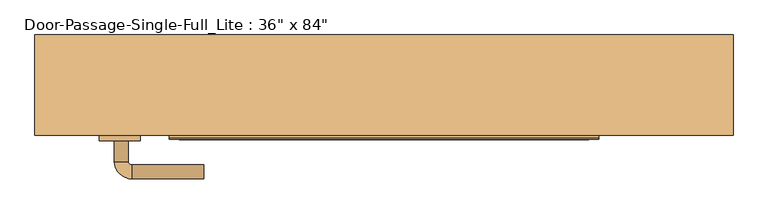
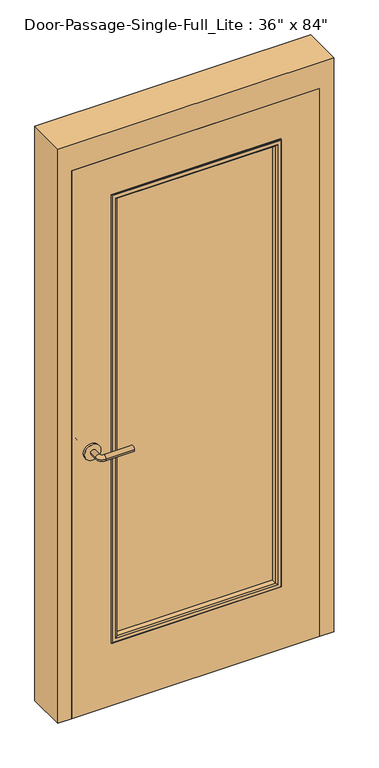
"""IFC4 building model written with IfcOpenShell, lengths in millimetres: door geometry."""

from ifc_helpers import new_model, si_unit, point, frame, frame_2d, origin, place, context, project, spatial, polyline, circle_curve, ellipse_curve, trimmed, segment, composite_curve, outline, extrude, faceted_brep, source, transform, mapped, element, save
from ifc_brep_helpers import plane_surface, cylinder_surface, revolved_surface, advanced_brep


def door_58f93f42(model_context):
    return source(origin(), model_context, "Body", "SolidModel", [
        advanced_brep(
        [(-392.190625, 1.65, 1016.0), (-372.190625, 1.65, 1016.0), (-392.190625, 31.65, 1016.0), (-372.190625, 31.65, 1016.0), (-367.190625, 36.65, 1016.0), (-367.190625, 56.65, 1016.0), (-262.190625, 56.65, 1016.0), (-262.190625, 36.65, 1016.0)],
        [
            (0, 1, circle_curve(frame((-382.190625, 1.65, 1016.0), z_axis=(0.0, -1.0, 0.0), x_axis=(1.0, 0.0, 0.0)), 10.0)),
            (1, 0, circle_curve(frame((-382.190625, 1.65, 1016.0), z_axis=(0.0, -1.0, 0.0), x_axis=(1.0, 0.0, 0.0)), 10.0)),
            (0, 2),
            (2, 3, circle_curve(frame((-382.190625, 31.65, 1016.0), z_axis=(0.0, -1.0, 0.0), x_axis=(1.0, 0.0, 0.0)), 10.0)),
            (3, 1),
            (3, 2, circle_curve(frame((-382.190625, 31.65, 1016.0), z_axis=(0.0, -1.0, 0.0), x_axis=(1.0, 0.0, 0.0)), 10.0)),
            (4, 3, circle_curve(frame((-367.190625, 31.65, 1016.0), z_axis=(0.0, 0.0, 1.0), x_axis=(-1.0, 0.0, 0.0)), 5.0)),
            (2, 5, circle_curve(frame((-367.190625, 31.65, 1016.0), z_axis=(0.0, 0.0, -1.0), x_axis=(-1.0, 0.0, 0.0)), 25.0)),
            (5, 4, circle_curve(frame((-367.190625, 46.65, 1016.0), z_axis=(-1.0, 0.0, 0.0), x_axis=(0.0, -1.0, 0.0)), 10.0)),
            (4, 5, circle_curve(frame((-367.190625, 46.65, 1016.0), z_axis=(-1.0, 0.0, 0.0), x_axis=(0.0, -1.0, 0.0)), 10.0)),
            (6, 7, circle_curve(frame((-262.190625, 46.65, 1016.0), z_axis=(1.0, 0.0, 0.0), x_axis=(0.0, -1.0, 0.0)), 10.0)),
            (7, 6, circle_curve(frame((-262.190625, 46.65, 1016.0), z_axis=(1.0, 0.0, 0.0), x_axis=(0.0, -1.0, 0.0)), 10.0)),
            (5, 6),
            (7, 4),
        ],
        [
            plane_surface(frame((-382.190625, 1.65, 1016.0), z_axis=(0.0, -1.0, 0.0), x_axis=(0.0, 0.0, 1.0))),
            cylinder_surface(frame((-382.190625, 1.65, 1016.0), z_axis=(0.0, -1.0, 0.0), x_axis=(1.0, 0.0, 0.0)), 10.0),
            revolved_surface(trimmed(ellipse_curve(frame((-382.190625, 31.65, 1016.0), z_axis=(0.0, -1.0, 0.0), x_axis=(1.0, 0.0, 0.0)), 10.0, 10.0), [point((-392.190625, 31.65, 1016.0))], [point((-372.190625, 31.65, 1016.0))], True, "CARTESIAN"), (-367.190625, 31.65, 1016.0), (0.0, 0.0, -1.0)),
            revolved_surface(trimmed(ellipse_curve(frame((-382.190625, 31.65, 1016.0), z_axis=(0.0, -1.0, 0.0), x_axis=(1.0, 0.0, 0.0)), 10.0, 10.0), [point((-372.190625, 31.65, 1016.0))], [point((-392.190625, 31.65, 1016.0))], True, "CARTESIAN"), (-367.190625, 31.65, 1016.0), (0.0, 0.0, -1.0)),
            plane_surface(frame((-262.190625, 46.65, 1016.0), z_axis=(1.0, 0.0, 0.0), x_axis=(0.0, 0.0, 1.0))),
            cylinder_surface(frame((-367.190625, 46.65, 1016.0), z_axis=(-1.0, 0.0, 0.0), x_axis=(0.0, -1.0, 0.0)), 10.0),
        ],
        [
            (0, [[1, 2]]),
            (1, [[-1, 3, 4, 5]]),
            (1, [[-2, -5, 6, -3]]),
            (2, [[7, -4, 8, 9]]),
            (3, [[-8, -6, -7, 10]]),
            (4, [[11, 12]]),
            (5, [[-9, 13, -12, 14]]),
            (5, [[-10, -14, -11, -13]]),
        ],
    ),
        extrude(outline(composite_curve([segment(trimmed(circle_curve(frame_2d((1016.0, -384.690625)), 30.0), [point((1016.0, -414.690625))], [point((1016.0, -354.690625))], False, "CARTESIAN"), True, "CONTINUOUS"), segment(trimmed(circle_curve(frame_2d((1016.0, -384.690625)), 30.0), [point((1016.0, -354.690625))], [point((1016.0, -414.690625))], False, "CARTESIAN"), True, "CONTINUOUS")], self_intersect=False)), frame((0.0, -6.35, 0.0), z_axis=(0.0, 1.0, 0.0), x_axis=(0.0, 0.0, 1.0)), (0.0, 0.0, 1.0), 8.0),
        advanced_brep(
        [(-392.190625, -58.8, 1016.0), (-372.190625, -58.8, 1016.0), (-372.190625, -88.8, 1016.0), (-392.190625, -88.8, 1016.0), (-367.190625, -93.8, 1016.0), (-367.190625, -113.8, 1016.0), (-262.190625, -113.8, 1016.0), (-262.190625, -93.8, 1016.0)],
        [
            (0, 1, circle_curve(frame((-382.190625, -58.8, 1016.0), z_axis=(0.0, 1.0, 0.0), x_axis=(1.0, 0.0, 0.0)), 10.0)),
            (1, 0, circle_curve(frame((-382.190625, -58.8, 1016.0), z_axis=(0.0, 1.0, 0.0), x_axis=(1.0, 0.0, 0.0)), 10.0)),
            (1, 2),
            (2, 3, circle_curve(frame((-382.190625, -88.8, 1016.0), z_axis=(0.0, 1.0, 0.0), x_axis=(1.0, 0.0, 0.0)), 10.0)),
            (3, 0),
            (3, 2, circle_curve(frame((-382.190625, -88.8, 1016.0), z_axis=(0.0, 1.0, 0.0), x_axis=(1.0, 0.0, 0.0)), 10.0)),
            (4, 5, circle_curve(frame((-367.190625, -103.8, 1016.0), z_axis=(-1.0, 0.0, 0.0), x_axis=(0.0, 1.0, 0.0)), 10.0)),
            (5, 3, circle_curve(frame((-367.190625, -88.8, 1016.0), z_axis=(0.0, 0.0, -1.0), x_axis=(-1.0, 0.0, 0.0)), 25.0)),
            (2, 4, circle_curve(frame((-367.190625, -88.8, 1016.0), z_axis=(0.0, 0.0, 1.0), x_axis=(-1.0, 0.0, 0.0)), 5.0)),
            (5, 4, circle_curve(frame((-367.190625, -103.8, 1016.0), z_axis=(-1.0, 0.0, 0.0), x_axis=(0.0, 1.0, 0.0)), 10.0)),
            (6, 7, circle_curve(frame((-262.190625, -103.8, 1016.0), z_axis=(1.0, 0.0, 0.0), x_axis=(0.0, 1.0, 0.0)), 10.0)),
            (7, 6, circle_curve(frame((-262.190625, -103.8, 1016.0), z_axis=(1.0, 0.0, 0.0), x_axis=(0.0, 1.0, 0.0)), 10.0)),
            (4, 7),
            (6, 5),
        ],
        [
            plane_surface(frame((-382.190625, -58.8, 1016.0), z_axis=(0.0, 1.0, 0.0), x_axis=(0.0, 0.0, 1.0))),
            cylinder_surface(frame((-382.190625, -58.8, 1016.0), z_axis=(0.0, 1.0, 0.0), x_axis=(1.0, 0.0, 0.0)), 10.0),
            revolved_surface(trimmed(ellipse_curve(frame((-382.190625, -88.8, 1016.0), z_axis=(0.0, -1.0, 0.0), x_axis=(1.0, 0.0, 0.0)), 10.0, 10.0), [point((-392.190625, -88.8, 1016.0))], [point((-372.190625, -88.8, 1016.0))], True, "CARTESIAN"), (-367.190625, -88.8, 1016.0), (0.0, 0.0, -1.0)),
            revolved_surface(trimmed(ellipse_curve(frame((-382.190625, -88.8, 1016.0), z_axis=(0.0, -1.0, 0.0), x_axis=(1.0, 0.0, 0.0)), 10.0, 10.0), [point((-372.190625, -88.8, 1016.0))], [point((-392.190625, -88.8, 1016.0))], True, "CARTESIAN"), (-367.190625, -88.8, 1016.0), (0.0, 0.0, -1.0)),
            plane_surface(frame((-262.190625, -103.8, 1016.0), z_axis=(1.0, 0.0, 0.0), x_axis=(0.0, 0.0, 1.0))),
            cylinder_surface(frame((-367.190625, -103.8, 1016.0), z_axis=(-1.0, 0.0, 0.0), x_axis=(0.0, 1.0, 0.0)), 10.0),
        ],
        [
            (0, [[1, 2]]),
            (1, [[3, 4, 5, -2]]),
            (1, [[-5, 6, -3, -1]]),
            (2, [[7, 8, -4, 9]]),
            (3, [[10, -9, -6, -8]]),
            (4, [[11, 12]]),
            (5, [[13, -11, 14, -7]]),
            (5, [[-14, -12, -13, -10]]),
        ],
    ),
        extrude(outline(composite_curve([segment(trimmed(circle_curve(frame_2d((1016.0, -384.690625)), 30.0), [point((1016.0, -414.690625))], [point((1016.0, -354.690625))], False, "CARTESIAN"), True, "CONTINUOUS"), segment(trimmed(circle_curve(frame_2d((1016.0, -384.690625)), 30.0), [point((1016.0, -354.690625))], [point((1016.0, -414.690625))], False, "CARTESIAN"), True, "CONTINUOUS")], self_intersect=False)), frame((0.0, -58.8, 0.0), z_axis=(0.0, 1.0, 0.0), x_axis=(0.0, 0.0, 1.0)), (0.0, 0.0, 1.0), 8.0),
        extrude(outline(polyline([(304.8, -25.4), (304.8, -31.75), (-304.8, -31.75), (-304.8, -25.4), (304.8, -25.4)])), frame((0.0, 0.0, 254.0), z_axis=(0.0, 0.0, 1.0), x_axis=(1.0, 0.0, 0.0)), (0.0, 0.0, 1.0), 1727.2),
        faceted_brep([(457.2, -1.5875, 0.0), (441.325, -1.5875, 0.0), (441.325, 46.0375, 0.0), (457.2, 46.0375, 0.0), (457.2, 95.25, 0.0), (508.0, 95.25, 0.0), (508.0, -50.8, 0.0), (457.2, -50.8, 0.0), (457.2, -50.8, 2133.6), (457.2, -1.5875, 2133.6), (508.0, -50.8, 2235.2), (-508.0, -50.8, 2235.2), (-508.0, -50.8, 0.0), (-457.2, -50.8, 0.0), (-457.2, -50.8, 2133.6), (508.0, 95.25, 2235.2), (457.2, 95.25, 2133.6), (-457.2, 95.25, 2133.6), (-457.2, 95.25, 0.0), (-508.0, 95.25, 0.0), (-508.0, 95.25, 2235.2), (457.2, 46.0375, 2133.6), (441.325, 46.0375, 2117.725), (-441.325, 46.0375, 2117.725), (-441.325, 46.0375, 0.0), (-457.2, 46.0375, 0.0), (-457.2, 46.0375, 2133.6), (441.325, -1.5875, 2117.725), (-457.2, -1.5875, 2133.6), (-457.2, -1.5875, 0.0), (-441.325, -1.5875, 0.0), (-441.325, -1.5875, 2117.725)], [[[0, 1, 2, 3, 4, 5, 6, 7]], [[7, 8, 9, 0]], [[6, 10, 11, 12, 13, 14, 8, 7]], [[5, 15, 10, 6]], [[4, 16, 17, 18, 19, 20, 15, 5]], [[3, 21, 16, 4]], [[2, 22, 23, 24, 25, 26, 21, 3]], [[1, 27, 22, 2]], [[0, 9, 28, 29, 30, 31, 27, 1]], [[8, 14, 28, 9]], [[16, 21, 26, 17]], [[22, 27, 31, 23]], [[12, 19, 18, 25, 24, 30, 29, 13]], [[13, 29, 28, 14]], [[11, 20, 19, 12]], [[17, 26, 25, 18]], [[23, 31, 30, 24]], [[15, 20, 11, 10]]]),
        extrude(outline(polyline([(2133.6, -457.2), (0.0, -457.2), (0.0, 457.2), (2133.6, 457.2), (2133.6, -457.2)]), holes=[polyline([(1981.2, -304.8), (1981.2, 304.8), (254.0, 304.8), (254.0, -304.8), (1981.2, -304.8)])]), frame((0.0, -50.8, 0.0), z_axis=(0.0, 1.0, 0.0), x_axis=(0.0, 0.0, 1.0)), (0.0, 0.0, 1.0), 44.45),
        advanced_brep(
        [(-304.8, -31.75, 1981.2), (-304.8, -31.75, 254.0), (-304.8, -50.8, 254.0), (-304.8, -50.8, 1981.2), (-292.8, -51.8, 1969.2), (-292.8, -51.8, 266.0), (-292.8, -31.75, 266.0), (-292.8, -31.75, 1969.2), (-297.8, -56.8, 1974.2), (-297.8, -56.8, 261.0), (-312.8, -54.8, 1989.2), (-312.8, -54.8, 246.0), (-310.8, -56.8, 248.0), (-310.8, -56.8, 1987.2), (-312.8, -50.8, 1989.2), (-312.8, -50.8, 246.0), (304.8, -31.75, 254.0), (304.8, -50.8, 254.0), (292.8, -51.8, 266.0), (292.8, -31.75, 266.0), (297.8, -56.8, 261.0), (312.8, -54.8, 246.0), (310.8, -56.8, 248.0), (312.8, -50.8, 246.0), (304.8, -31.75, 1981.2), (304.8, -50.8, 1981.2), (292.8, -51.8, 1969.2), (292.8, -31.75, 1969.2), (297.8, -56.8, 1974.2), (312.8, -54.8, 1989.2), (310.8, -56.8, 1987.2), (312.8, -50.8, 1989.2)],
        [
            (0, 1),
            (1, 2),
            (2, 3),
            (3, 0),
            (4, 5),
            (5, 6),
            (6, 7),
            (7, 4),
            (8, 9),
            (9, 5, ellipse_curve(frame((-297.8, -51.8, 261.0), z_axis=(-0.7071067811865475, 0.0, 0.7071067811865475), x_axis=(0.7071067811865474, 0.0, 0.7071067811865476)), 7.0710678, 5.0)),
            (4, 8, ellipse_curve(frame((-297.8, -51.8, 1974.2), z_axis=(-0.7071067811865475, 0.0, -0.7071067811865475), x_axis=(-0.7071067811865474, 0.0, 0.7071067811865476)), 7.0710678, 5.0)),
            (10, 11),
            (11, 12, ellipse_curve(frame((-310.8, -54.8, 248.0), z_axis=(-0.7071067811865475, 0.0, 0.7071067811865475), x_axis=(0.7071067811865474, 0.0, 0.7071067811865476)), 2.8284271, 2.0)),
            (12, 13),
            (13, 10, ellipse_curve(frame((-310.8, -54.8, 1987.2), z_axis=(-0.7071067811865475, 0.0, -0.7071067811865475), x_axis=(-0.7071067811865474, 0.0, 0.7071067811865476)), 2.8284271, 2.0)),
            (14, 15),
            (15, 11),
            (10, 14),
            (1, 16),
            (16, 17),
            (17, 2),
            (5, 18),
            (18, 19),
            (19, 6),
            (9, 20),
            (20, 18, ellipse_curve(frame((297.8, -51.8, 261.0), z_axis=(-0.7071067811865475, 0.0, -0.7071067811865475), x_axis=(-0.7071067811865476, 0.0, 0.7071067811865474)), 7.0710678, 5.0)),
            (11, 21),
            (21, 22, ellipse_curve(frame((310.8, -54.8, 248.0), z_axis=(-0.7071067811865475, 0.0, -0.7071067811865475), x_axis=(-0.7071067811865476, 0.0, 0.7071067811865474)), 2.8284271, 2.0)),
            (22, 12),
            (15, 23),
            (23, 21),
            (16, 24),
            (24, 25),
            (25, 17),
            (18, 26),
            (26, 27),
            (27, 19),
            (20, 28),
            (28, 26, ellipse_curve(frame((297.8, -51.8, 1974.2), z_axis=(0.7071067811865475, 0.0, -0.7071067811865475), x_axis=(-0.7071067811865474, 0.0, -0.7071067811865476)), 7.0710678, 5.0)),
            (21, 29),
            (29, 30, ellipse_curve(frame((310.8, -54.8, 1987.2), z_axis=(0.7071067811865475, 0.0, -0.7071067811865475), x_axis=(-0.7071067811865474, 0.0, -0.7071067811865476)), 2.8284271, 2.0)),
            (30, 22),
            (23, 31),
            (31, 29),
            (14, 31),
            (25, 3),
            (24, 0),
            (27, 7),
            (26, 4),
            (28, 8),
            (30, 13),
            (29, 10),
        ],
        [
            plane_surface(frame((-304.8, -50.8, 1981.2), z_axis=(-1.0, 0.0, 0.0), x_axis=(0.0, 0.0, -1.0))),
            plane_surface(frame((-292.8, -31.75, 1969.2), z_axis=(1.0, 0.0, 0.0), x_axis=(0.0, 0.0, -1.0))),
            cylinder_surface(frame((-297.8, -51.8, 1981.2), z_axis=(0.0, 0.0, 1.0), x_axis=(-1.0, 0.0, 0.0)), 5.0),
            cylinder_surface(frame((-310.8, -54.8, 1981.2), z_axis=(0.0, 0.0, 1.0), x_axis=(-1.0, 0.0, 0.0)), 2.0),
            plane_surface(frame((-312.8, -54.8, 1989.2), z_axis=(-1.0, 0.0, 0.0), x_axis=(0.0, 0.0, -1.0))),
            plane_surface(frame((-304.8, -50.8, 254.0), z_axis=(0.0, 0.0, -1.0), x_axis=(1.0, 0.0, 0.0))),
            plane_surface(frame((-292.8, -31.75, 266.0), z_axis=(0.0, 0.0, 1.0), x_axis=(1.0, 0.0, 0.0))),
            cylinder_surface(frame((-304.8, -51.8, 261.0), z_axis=(-1.0, 0.0, 0.0), x_axis=(0.0, 0.0, -1.0)), 5.0),
            cylinder_surface(frame((-304.8, -54.8, 248.0), z_axis=(-1.0, 0.0, 0.0), x_axis=(0.0, 0.0, -1.0)), 2.0),
            plane_surface(frame((-312.8, -54.8, 246.0), z_axis=(0.0, 0.0, -1.0), x_axis=(1.0, 0.0, 0.0))),
            plane_surface(frame((304.8, -50.8, 254.0), z_axis=(1.0, 0.0, 0.0), x_axis=(0.0, 0.0, 1.0))),
            plane_surface(frame((292.8, -31.75, 266.0), z_axis=(-1.0, 0.0, 0.0), x_axis=(0.0, 0.0, 1.0))),
            cylinder_surface(frame((297.8, -51.8, 254.0), z_axis=(0.0, 0.0, -1.0), x_axis=(1.0, 0.0, 0.0)), 5.0),
            cylinder_surface(frame((310.8, -54.8, 254.0), z_axis=(0.0, 0.0, -1.0), x_axis=(1.0, 0.0, 0.0)), 2.0),
            plane_surface(frame((312.8, -54.8, 246.0), z_axis=(1.0, 0.0, 0.0), x_axis=(0.0, 0.0, 1.0))),
            plane_surface(frame((312.8, -50.8, 1989.2), z_axis=(0.0, 1.0, 0.0), x_axis=(-1.0, 0.0, 0.0))),
            plane_surface(frame((304.8, -50.8, 1981.2), z_axis=(0.0, 0.0, 1.0), x_axis=(-1.0, 0.0, 0.0))),
            plane_surface(frame((304.8, -31.75, 1981.2), z_axis=(0.0, 1.0, 0.0), x_axis=(-1.0, 0.0, 0.0))),
            plane_surface(frame((292.8, -31.75, 1969.2), z_axis=(0.0, 0.0, -1.0), x_axis=(-1.0, 0.0, 0.0))),
            cylinder_surface(frame((304.8, -51.8, 1974.2), z_axis=(1.0, 0.0, 0.0), x_axis=(0.0, 0.0, 1.0)), 5.0),
            plane_surface(frame((297.8, -56.8, 1974.2), z_axis=(0.0, -1.0, 0.0), x_axis=(-1.0, 0.0, 0.0))),
            cylinder_surface(frame((304.8, -54.8, 1987.2), z_axis=(1.0, 0.0, 0.0), x_axis=(0.0, 0.0, 1.0)), 2.0),
            plane_surface(frame((312.8, -54.8, 1989.2), z_axis=(0.0, 0.0, 1.0), x_axis=(-1.0, 0.0, 0.0))),
        ],
        [
            (0, [[1, 2, 3, 4]]),
            (1, [[5, 6, 7, 8]]),
            (2, [[9, 10, -5, 11]]),
            (3, [[12, 13, 14, 15]]),
            (4, [[16, 17, -12, 18]]),
            (5, [[19, 20, 21, -2]]),
            (6, [[22, 23, 24, -6]]),
            (7, [[25, 26, -22, -10]]),
            (8, [[27, 28, 29, -13]]),
            (9, [[30, 31, -27, -17]]),
            (10, [[32, 33, 34, -20]]),
            (11, [[35, 36, 37, -23]]),
            (12, [[38, 39, -35, -26]]),
            (13, [[40, 41, 42, -28]]),
            (14, [[43, 44, -40, -31]]),
            (15, [[-16, 45, -43, -30], [-3, -21, -34, 46]]),
            (16, [[47, -4, -46, -33]]),
            (17, [[-1, -47, -32, -19], [-7, -24, -37, 48]]),
            (18, [[49, -8, -48, -36]]),
            (19, [[50, -11, -49, -39]]),
            (20, [[-14, -29, -42, 51], [-9, -50, -38, -25]]),
            (21, [[52, -15, -51, -41]]),
            (22, [[-45, -18, -52, -44]]),
        ],
    ),
        advanced_brep(
        [(-304.8, -25.4, 254.0), (-304.8, -25.4, 1981.2), (-304.8, -6.35, 1981.2), (-304.8, -6.35, 254.0), (-292.8, -5.35, 266.0), (-292.8, -5.35, 1969.2), (-292.8, -25.4, 1969.2), (-292.8, -25.4, 266.0), (-297.8, -0.35, 261.0), (-297.8, -0.35, 1974.2), (-312.8, -2.35, 246.0), (-312.8, -2.35, 1989.2), (-310.8, -0.35, 1987.2), (-310.8, -0.35, 248.0), (-312.8, -6.35, 246.0), (-312.8, -6.35, 1989.2), (304.8, -25.4, 1981.2), (304.8, -6.35, 1981.2), (292.8, -5.35, 1969.2), (292.8, -25.4, 1969.2), (297.8, -0.35, 1974.2), (312.8, -2.35, 1989.2), (310.8, -0.35, 1987.2), (312.8, -6.35, 1989.2), (304.8, -25.4, 254.0), (304.8, -6.35, 254.0), (292.8, -5.35, 266.0), (292.8, -25.4, 266.0), (297.8, -0.35, 261.0), (312.8, -2.35, 246.0), (310.8, -0.35, 248.0), (312.8, -6.35, 246.0)],
        [
            (0, 1),
            (1, 2),
            (2, 3),
            (3, 0),
            (4, 5),
            (5, 6),
            (6, 7),
            (7, 4),
            (8, 9),
            (9, 5, ellipse_curve(frame((-297.8, -5.35, 1974.2), z_axis=(-0.7071067811865475, 0.0, -0.7071067811865475), x_axis=(0.7071067811865474, 0.0, -0.7071067811865476)), 7.0710678, 5.0)),
            (4, 8, ellipse_curve(frame((-297.8, -5.35, 261.0), z_axis=(-0.7071067811865475, 0.0, 0.7071067811865475), x_axis=(-0.7071067811865474, 0.0, -0.7071067811865476)), 7.0710678, 5.0)),
            (10, 11),
            (11, 12, ellipse_curve(frame((-310.8, -2.35, 1987.2), z_axis=(-0.7071067811865475, 0.0, -0.7071067811865475), x_axis=(0.7071067811865474, 0.0, -0.7071067811865476)), 2.8284271, 2.0)),
            (12, 13),
            (13, 10, ellipse_curve(frame((-310.8, -2.35, 248.0), z_axis=(-0.7071067811865475, 0.0, 0.7071067811865475), x_axis=(-0.7071067811865474, 0.0, -0.7071067811865476)), 2.8284271, 2.0)),
            (14, 15),
            (15, 11),
            (10, 14),
            (1, 16),
            (16, 17),
            (17, 2),
            (5, 18),
            (18, 19),
            (19, 6),
            (9, 20),
            (20, 18, ellipse_curve(frame((297.8, -5.35, 1974.2), z_axis=(-0.7071067811865475, 0.0, 0.7071067811865475), x_axis=(-0.7071067811865476, 0.0, -0.7071067811865474)), 7.0710678, 5.0)),
            (11, 21),
            (21, 22, ellipse_curve(frame((310.8, -2.35, 1987.2), z_axis=(-0.7071067811865475, 0.0, 0.7071067811865475), x_axis=(-0.7071067811865476, 0.0, -0.7071067811865474)), 2.8284271, 2.0)),
            (22, 12),
            (15, 23),
            (23, 21),
            (16, 24),
            (24, 25),
            (25, 17),
            (18, 26),
            (26, 27),
            (27, 19),
            (20, 28),
            (28, 26, ellipse_curve(frame((297.8, -5.35, 261.0), z_axis=(0.7071067811865475, 0.0, 0.7071067811865475), x_axis=(-0.7071067811865474, 0.0, 0.7071067811865476)), 7.0710678, 5.0)),
            (21, 29),
            (29, 30, ellipse_curve(frame((310.8, -2.35, 248.0), z_axis=(0.7071067811865475, 0.0, 0.7071067811865475), x_axis=(-0.7071067811865474, 0.0, 0.7071067811865476)), 2.8284271, 2.0)),
            (30, 22),
            (23, 31),
            (31, 29),
            (14, 31),
            (25, 3),
            (24, 0),
            (27, 7),
            (26, 4),
            (28, 8),
            (30, 13),
            (29, 10),
        ],
        [
            plane_surface(frame((-304.8, -6.35, 254.0), z_axis=(-1.0, 0.0, 0.0), x_axis=(0.0, 0.0, 1.0))),
            plane_surface(frame((-292.8, -25.4, 266.0), z_axis=(1.0, 0.0, 0.0), x_axis=(0.0, 0.0, 1.0))),
            cylinder_surface(frame((-297.8, -5.35, 254.0), z_axis=(0.0, 0.0, -1.0), x_axis=(-1.0, 0.0, 0.0)), 5.0),
            cylinder_surface(frame((-310.8, -2.35, 254.0), z_axis=(0.0, 0.0, -1.0), x_axis=(-1.0, 0.0, 0.0)), 2.0),
            plane_surface(frame((-312.8, -2.35, 246.0), z_axis=(-1.0, 0.0, 0.0), x_axis=(0.0, 0.0, 1.0))),
            plane_surface(frame((-304.8, -6.35, 1981.2), z_axis=(0.0, 0.0, 1.0), x_axis=(1.0, 0.0, 0.0))),
            plane_surface(frame((-292.8, -25.4, 1969.2), z_axis=(0.0, 0.0, -1.0), x_axis=(1.0, 0.0, 0.0))),
            cylinder_surface(frame((-304.8, -5.35, 1974.2), z_axis=(-1.0, 0.0, 0.0), x_axis=(0.0, 0.0, 1.0)), 5.0),
            cylinder_surface(frame((-304.8, -2.35, 1987.2), z_axis=(-1.0, 0.0, 0.0), x_axis=(0.0, 0.0, 1.0)), 2.0),
            plane_surface(frame((-312.8, -2.35, 1989.2), z_axis=(0.0, 0.0, 1.0), x_axis=(1.0, 0.0, 0.0))),
            plane_surface(frame((304.8, -6.35, 1981.2), z_axis=(1.0, 0.0, 0.0), x_axis=(0.0, 0.0, -1.0))),
            plane_surface(frame((292.8, -25.4, 1969.2), z_axis=(-1.0, 0.0, 0.0), x_axis=(0.0, 0.0, -1.0))),
            cylinder_surface(frame((297.8, -5.35, 1981.2), z_axis=(0.0, 0.0, 1.0), x_axis=(1.0, 0.0, 0.0)), 5.0),
            cylinder_surface(frame((310.8, -2.35, 1981.2), z_axis=(0.0, 0.0, 1.0), x_axis=(1.0, 0.0, 0.0)), 2.0),
            plane_surface(frame((312.8, -2.35, 1989.2), z_axis=(1.0, 0.0, 0.0), x_axis=(0.0, 0.0, -1.0))),
            plane_surface(frame((312.8, -6.35, 246.0), z_axis=(0.0, -1.0, 0.0), x_axis=(-1.0, 0.0, 0.0))),
            plane_surface(frame((304.8, -6.35, 254.0), z_axis=(0.0, 0.0, -1.0), x_axis=(-1.0, 0.0, 0.0))),
            plane_surface(frame((304.8, -25.4, 254.0), z_axis=(0.0, -1.0, 0.0), x_axis=(-1.0, 0.0, 0.0))),
            plane_surface(frame((292.8, -25.4, 266.0), z_axis=(0.0, 0.0, 1.0), x_axis=(-1.0, 0.0, 0.0))),
            cylinder_surface(frame((304.8, -5.35, 261.0), z_axis=(1.0, 0.0, 0.0), x_axis=(0.0, 0.0, -1.0)), 5.0),
            plane_surface(frame((297.8, -0.35, 261.0), z_axis=(0.0, 1.0, 0.0), x_axis=(-1.0, 0.0, 0.0))),
            cylinder_surface(frame((304.8, -2.35, 248.0), z_axis=(1.0, 0.0, 0.0), x_axis=(0.0, 0.0, -1.0)), 2.0),
            plane_surface(frame((312.8, -2.35, 246.0), z_axis=(0.0, 0.0, -1.0), x_axis=(-1.0, 0.0, 0.0))),
        ],
        [
            (0, [[1, 2, 3, 4]]),
            (1, [[5, 6, 7, 8]]),
            (2, [[9, 10, -5, 11]]),
            (3, [[12, 13, 14, 15]]),
            (4, [[16, 17, -12, 18]]),
            (5, [[19, 20, 21, -2]]),
            (6, [[22, 23, 24, -6]]),
            (7, [[25, 26, -22, -10]]),
            (8, [[27, 28, 29, -13]]),
            (9, [[30, 31, -27, -17]]),
            (10, [[32, 33, 34, -20]]),
            (11, [[35, 36, 37, -23]]),
            (12, [[38, 39, -35, -26]]),
            (13, [[40, 41, 42, -28]]),
            (14, [[43, 44, -40, -31]]),
            (15, [[-16, 45, -43, -30], [-3, -21, -34, 46]]),
            (16, [[47, -4, -46, -33]]),
            (17, [[-1, -47, -32, -19], [-7, -24, -37, 48]]),
            (18, [[49, -8, -48, -36]]),
            (19, [[50, -11, -49, -39]]),
            (20, [[-14, -29, -42, 51], [-9, -50, -38, -25]]),
            (21, [[52, -15, -51, -41]]),
            (22, [[-45, -18, -52, -44]]),
        ],
    ),
    ])


if __name__ == "__main__":
    model = new_model("IFC4")
    model_context = context("Model", 3, world=origin())
    ifc_project = project(units=[si_unit("LENGTHUNIT", "METRE", prefix="MILLI")], contexts=[model_context])
    site = spatial("IfcSite", under=ifc_project)
    building = spatial("IfcBuilding", under=site)
    placement = place(None, origin())
    door_shape = door_58f93f42(model_context)
    element("IfcDoor", 1, ObjectType="Door-Passage-Single-Full_Lite : 36\" x 84\"", at=placement, inside=building, context=model_context, shape_type="MappedRepresentation", body=[
        mapped(door_shape, transform((0.0, 0.0, 0.0), x_axis=(1.0, 0.0, 0.0), y_axis=(0.0, 1.0, 0.0), z_axis=(0.0, 0.0, 1.0))),
    ])
    save(model, "model.ifc")

# Revit data of these elements
# Type "Door-Passage-Single-Full_Lite : 36\" x 84\""
#   Type Mark = "52"
#   Assembly Code = "B2030100"
#   Analytic Construction = "Wooden"
#   Thickness = 0' - 1 3/4"
#   Thermal Resistance (R) = 2.5876 (h·ft²·°F)/BTU
#   Swing Angle [instance default] = 90.00°
#   Strike Height = 3' - 4"
#   Rough Width [instance default] = 3' - 4"
#   Rough Height [instance default] = 7' - 4"
#   MF Opening Height [instance default] = 0' - 4"
#   MF Opening Width [instance default] = 0' - 4"
#   Inset Calculate [instance default] = 0' - 4"
#   Masonry Inset [instance default] = 0' - 1"
#   Height = 7' - 0"
#   Width = 3' - 0"
#   Heat Transfer Coefficient (U) = 0.3865 BTU/(h·ft²·°F)
#   Masonry Frame Depth = 0' - 5 3/4"
#   Masonry Frame [instance default] = yes
#   Function = 1
#   Dry Wall Frame [instance default] = no
#   Panel Material = Wood - Birch
#   Glazing = Glass
#   Glass Stop Material = Metal - Paint Finish - Grey
#   Frame Material = Metal - Paint Finish - Grey
#   Door Handle Material = Aluminum
#   Visual Light Transmittance = 0
#   Solar Heat Gain Coefficient = 0
#   Wall Closure = (empty or 0)
# Element 1 (IfcDoor, "Door-Passage-Single-Full_Lite : 36\" x 84\"")
#   Materials on its faces: "Metal - Paint Finish - Grey", "Aluminum", "Wood - Birch", "Glass"
# Materials
#   "Wood - Birch": class "Wood", colour RGB 166 116 52, transparency 0, Cost = 0
#   "Glass": class "Glass", colour RGB 0 128 192, transparency 0.75, Description = "Soda Lime Glass", Cost = 0
#   "Metal - Paint Finish - Grey": class "Paint", colour RGB 104 104 104, transparency 0, Cost = 0
#   "Aluminum": class "Metal", colour RGB 247 247 247, transparency 0, Description = "Aluminum 6061", Cost = 0
